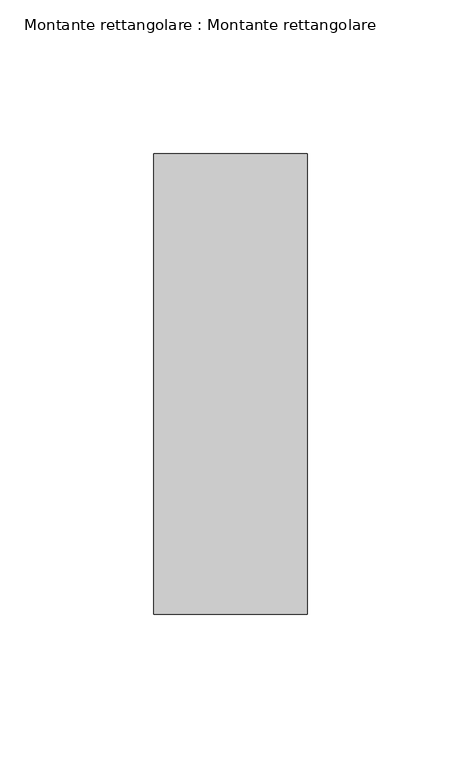
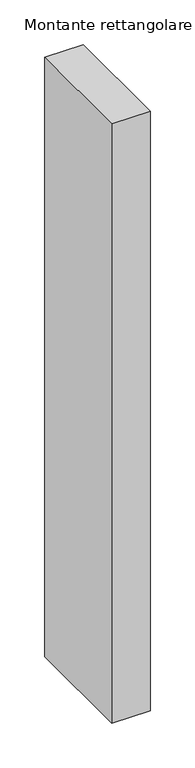
"""IFC4 building model written with IfcOpenShell, lengths in millimetres: member geometry, Montante rettangolare : Montante rettangolare."""

import ifcopenshell
import ifcopenshell.guid

model = None  # the IFC model being written
_history = None  # IfcOwnerHistory: only IFC2X3 demands one
_inside = {}  # id of a spatial element -> (the spatial element, [elements in it])
_under = {}  # id of a project, library or spatial element -> (it, [spatial elements below it])
_declared = {}  # id of a project -> (the project, [libraries it declares])
_typed = {}  # id of a type object -> (the type object, [elements of that type])
_made_of = {}  # id of a material, layer set ... -> (it, [elements and type objects made of it])


def new_model(schema):
    """Start an empty IFC model of exactly this schema.

    Asked for "IFC4X3", IfcOpenShell would pick the latest addendum, in which some entities
    have other attributes; the version numbers below select the first issue.
    IFC2X3 requires an IfcOwnerHistory on every rooted entity: one is made here for all.
    """
    global model, _history
    if schema == "IFC4X3":
        model = ifcopenshell.file(schema_version=(4, 3, 0, 0))
    else:
        model = ifcopenshell.file(schema=schema)
    _inside.clear()
    _under.clear()
    _declared.clear()
    _typed.clear()
    _made_of.clear()
    _history = None
    if model.schema == "IFC2X3":
        org = make("IfcOrganization", Name="unknown")
        user = make(
            "IfcPersonAndOrganization",
            ThePerson=make("IfcPerson", FamilyName="unknown"),
            TheOrganization=org,
        )
        app = make(
            "IfcApplication",
            ApplicationDeveloper=org,
            Version="unknown",
            ApplicationFullName="unknown",
            ApplicationIdentifier="unknown",
        )
        _history = make(
            "IfcOwnerHistory",
            OwningUser=user,
            OwningApplication=app,
            ChangeAction="ADDED",
            CreationDate=0,
        )
    return model


def make(cls, **values):
    """One entity of the class cls with the attributes given. An attribute that is None is left unset."""
    return model.create_entity(
        cls, **{name: value for name, value in values.items() if value is not None}
    )


def rooted(cls, **values):
    """An entity with a GlobalId (a new one), such as an element, a storey or a relation."""
    return make(cls, GlobalId=ifcopenshell.guid.new(), OwnerHistory=_history, **values)


def si_unit(unit_type, name, prefix=None):
    """IfcSIUnit, for example si_unit("LENGTHUNIT", "METRE", prefix="MILLI")."""
    return make("IfcSIUnit", UnitType=unit_type, Prefix=prefix, Name=name)


def assignment(units):
    """IfcUnitAssignment: the units of a project."""
    return None if units is None else make("IfcUnitAssignment", Units=units)


def point(xyz):
    """IfcCartesianPoint."""
    return None if xyz is None else make("IfcCartesianPoint", Coordinates=xyz)


def direction(xyz):
    """IfcDirection."""
    return None if xyz is None else make("IfcDirection", DirectionRatios=xyz)


def frame(location, z_axis=None, x_axis=None):
    """IfcAxis2Placement3D, a coordinate frame: its origin and axes. An axis left out is left unset."""
    return make(
        "IfcAxis2Placement3D",
        Location=point(location),
        Axis=direction(z_axis),
        RefDirection=direction(x_axis),
    )


def origin():
    """The frame at (0, 0, 0) with its axes left unset."""
    return frame((0.0, 0.0, 0.0))


def place(relative_to, where):
    """IfcLocalPlacement: puts the frame where relative to a parent placement (None: the world)."""
    return make(
        "IfcLocalPlacement", PlacementRelTo=relative_to, RelativePlacement=where
    )


def context(
    kind, dimensions, precision=None, world=None, true_north=None, identifier=None
):
    """IfcGeometricRepresentationContext, for example the 3D "Model" context."""
    return make(
        "IfcGeometricRepresentationContext",
        ContextIdentifier=identifier,
        ContextType=kind,
        CoordinateSpaceDimension=dimensions,
        Precision=precision,
        WorldCoordinateSystem=world,
        TrueNorth=true_north,
    )


def project(units=None, contexts=None):
    """IfcProject with its units and contexts."""
    return rooted(
        "IfcProject",
        Name="project",
        RepresentationContexts=contexts,
        UnitsInContext=assignment(units),
    )


def spatial(cls, under=None, at=None, **own):
    """A site, building, storey or space (cls), placed at a placement, below another one or the project."""
    s = rooted(cls, ObjectPlacement=at, **own)
    if under is not None:
        _under.setdefault(under.id(), (under, []))[1].append(s)
    return s


def polyline(points):
    """IfcPolyline through the points."""
    return make("IfcPolyline", Points=[point(p) for p in points])


def outline(outer, holes=None, kind="AREA"):
    """IfcArbitraryClosedProfileDef: a profile drawn as a closed curve; with holes, ...WithVoids."""
    if holes is None:
        return make("IfcArbitraryClosedProfileDef", ProfileType=kind, OuterCurve=outer)
    return make(
        "IfcArbitraryProfileDefWithVoids",
        ProfileType=kind,
        OuterCurve=outer,
        InnerCurves=holes,
    )


def extrude(swept, where, along, depth):
    """IfcExtrudedAreaSolid: the profile swept, set in the frame where, extruded along a direction by depth."""
    return make(
        "IfcExtrudedAreaSolid",
        SweptArea=swept,
        Position=where,
        ExtrudedDirection=direction(along),
        Depth=depth,
    )


def shape(context_of_items, identifier, shape_type, items):
    """IfcShapeRepresentation: the items that make up one representation, for example the "Body"."""
    return make(
        "IfcShapeRepresentation",
        ContextOfItems=context_of_items,
        RepresentationIdentifier=identifier,
        RepresentationType=shape_type,
        Items=items,
    )


def source(mapping_origin, context_of_items, identifier, shape_type, items):
    """IfcRepresentationMap: a shape defined once, which mapped items show again and again."""
    return make(
        "IfcRepresentationMap",
        MappingOrigin=mapping_origin,
        MappedRepresentation=shape(context_of_items, identifier, shape_type, items),
    )


def transform(
    local_origin,
    x_axis=None,
    y_axis=None,
    z_axis=None,
    scale=None,
    scale2=None,
    scale3=None,
    uniform=True,
):
    """IfcCartesianTransformationOperator3D, or its non-uniform kind. x_axis, y_axis, z_axis: its Axis1, 2, 3."""
    if uniform:
        return make(
            "IfcCartesianTransformationOperator3D",
            Axis1=direction(x_axis),
            Axis2=direction(y_axis),
            LocalOrigin=point(local_origin),
            Scale=scale,
            Axis3=direction(z_axis),
        )
    return make(
        "IfcCartesianTransformationOperator3DnonUniform",
        Axis1=direction(x_axis),
        Axis2=direction(y_axis),
        LocalOrigin=point(local_origin),
        Scale=scale,
        Axis3=direction(z_axis),
        Scale2=scale2,
        Scale3=scale3,
    )


def mapped(mapping_source, mapping_target):
    """IfcMappedItem: shows the shape of a source again, moved by a transform."""
    return make(
        "IfcMappedItem", MappingSource=mapping_source, MappingTarget=mapping_target
    )


def made_of(thing, what):
    """Note that an element or type object is made of a material, layer set ...; save() writes the relation."""
    if what is not None:
        _made_of.setdefault(what.id(), (what, []))[1].append(thing)
    return thing


def element(
    cls,
    number,
    at=None,
    inside=None,
    cuts=None,
    type_object=None,
    material=None,
    context=None,
    identifier="Body",
    shape_type=None,
    held_by="IfcProductDefinitionShape",
    body=None,
    shapes=None,
    **own,
):
    """One element of the class cls, such as IfcWall. Its Tag is "e" and its number.

    at: its placement. inside: the storey or other place that contains it. cuts: it is an
    opening in that element (IfcRelVoidsElement). A single representation is given by context,
    identifier, shape_type and body (its items); several are given by shapes. held_by: the class
    of the entity that holds the representations. save() writes the other relations.
    """
    e = rooted(cls, Tag="e%d" % number, ObjectPlacement=at, **own)
    if body is not None:
        shapes = [shape(context, identifier, shape_type, body)]
    if shapes is not None:
        e.Representation = make(held_by, Representations=shapes)
    if inside is not None:
        _inside.setdefault(inside.id(), (inside, []))[1].append(e)
    if cuts is not None:
        rooted(
            "IfcRelVoidsElement", RelatingBuildingElement=cuts, RelatedOpeningElement=e
        )
    if type_object is not None:
        _typed.setdefault(type_object.id(), (type_object, []))[1].append(e)
    return made_of(e, material)


def aggregate(whole, parts):
    """IfcRelAggregates: a whole, such as a stair, and the parts it consists of."""
    return rooted("IfcRelAggregates", RelatingObject=whole, RelatedObjects=parts)


def save(model, path):
    """Write the relations noted so far, then the file.

    IfcRelAggregates (storeys below a building ...), IfcRelContainedInSpatialStructure (elements
    in a storey), IfcRelDefinesByType, IfcRelAssociatesMaterial and IfcRelDeclares: one each for
    every whole, place, type object, material and project.
    """
    for whole, parts in _under.values():
        aggregate(whole, parts)
    for where, things in _inside.values():
        rooted(
            "IfcRelContainedInSpatialStructure",
            RelatedElements=things,
            RelatingStructure=where,
        )
    for kind, things in _typed.values():
        rooted("IfcRelDefinesByType", RelatedObjects=things, RelatingType=kind)
    for what, things in _made_of.values():
        rooted("IfcRelAssociatesMaterial", RelatedObjects=things, RelatingMaterial=what)
    for by, libraries in _declared.values():
        rooted("IfcRelDeclares", RelatingContext=by, RelatedDefinitions=libraries)
    model.write(path)


def montante_rettangolare_montante_rettangolare_14e9e993(model_context):
    return source(origin(), model_context, "Body", "SweptSolid", [
        extrude(outline(polyline([(25.0, 75.0), (25.0, -75.0), (-25.0, -75.0), (-25.0, 75.0), (25.0, 75.0)])), frame((0.0, 0.0, -820.0), z_axis=(0.0, 0.0, 1.0), x_axis=(1.0, 0.0, 0.0)), (0.0, 0.0, 1.0), 820.0),
    ])


if __name__ == "__main__":
    model = new_model("IFC4")
    model_context = context("Model", 3, world=origin())
    ifc_project = project(units=[si_unit("LENGTHUNIT", "METRE", prefix="MILLI")], contexts=[model_context])
    site = spatial("IfcSite", under=ifc_project)
    building = spatial("IfcBuilding", under=site)
    placement = place(None, origin())
    montante_rettangolare_montante_rettangolare_shape = montante_rettangolare_montante_rettangolare_14e9e993(model_context)
    element("IfcMember", 1, ObjectType="Montante rettangolare : Montante rettangolare", at=placement, inside=building, context=model_context, shape_type="MappedRepresentation", body=[
        mapped(montante_rettangolare_montante_rettangolare_shape, transform((0.0, 0.0, 0.0), x_axis=(1.0, 0.0, 0.0), y_axis=(0.0, 1.0, 0.0), z_axis=(0.0, 0.0, 1.0))),
    ])
    save(model, "model.ifc")

# Revit data of these elements
# Type "Montante rettangolare : Montante rettangolare"
#   built-in parameter 1007304 = 0.492126 (stored number, unit not read)
#   built-in parameter 1007301 = 0.082021 (stored number, unit not read)
#   built-in parameter 1007300 = 0.082021 (stored number, unit not read)
# Element 1 (IfcMember, "Montante rettangolare : Montante rettangolare")
#   Materials on its faces: "Acciaio"
# Materials
#   "Acciaio": class "Metallo", colour RGB 247 247 247, transparency 0, Description = "Acciaio, finitura zigrinata", Cost = 0
